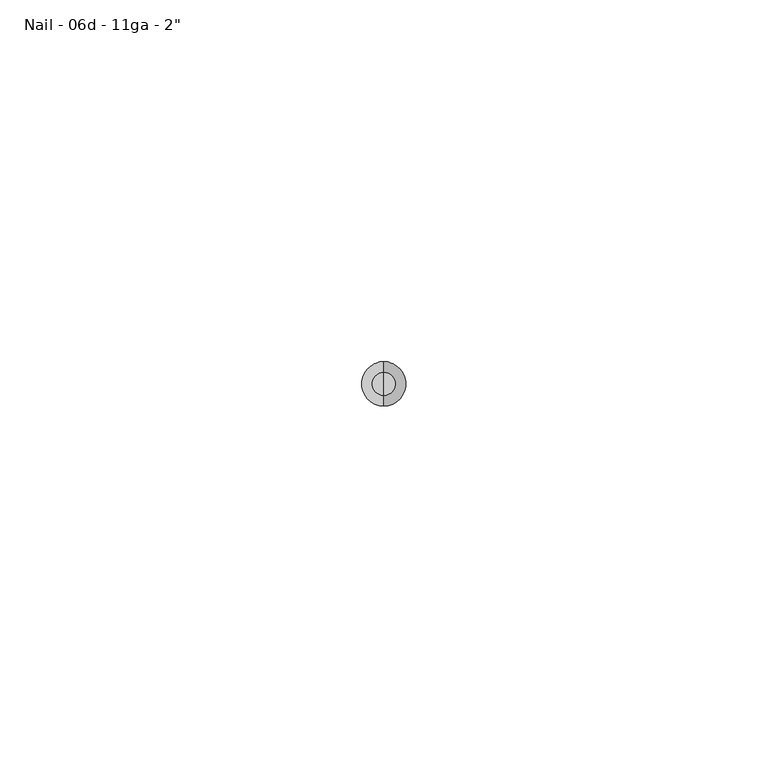
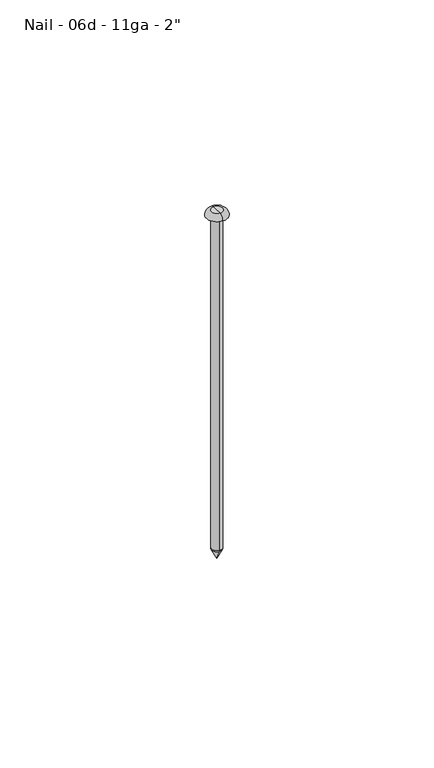
"""IFC4 building model written with IfcOpenShell, lengths in millimetres: fastener geometry."""

from ifc_helpers import new_model, si_unit, point, frame, origin, origin_2d, place, context, project, spatial, polyline, circle_curve, ellipse_curve, trimmed, segment, composite_curve, outline, extrude, source, transform, mapped, element, save
from ifc_brep_helpers import plane_surface, revolved_surface, advanced_brep


def fastener_73949ac7(model_context):
    return source(origin(), model_context, "Body", "SolidModel", [
        advanced_brep(
        [(0.0, -1.524, -101.6), (0.0, 1.524, -101.6), (0.0, 0.0, -101.6), (0.0, 0.0, -104.648)],
        [
            (0, 1, circle_curve(frame((0.0, 0.0, -101.6), z_axis=(0.0, 0.0, 1.0), x_axis=(0.0, 1.0, 0.0)), 1.524)),
            (1, 2),
            (2, 0),
            (1, 0, circle_curve(frame((0.0, 0.0, -101.6), z_axis=(0.0, 0.0, 1.0), x_axis=(0.0, 1.0, 0.0)), 1.524)),
            (3, 1),
            (0, 3),
        ],
        [
            plane_surface(frame((0.0, 0.0, -101.6), z_axis=(0.0, 0.0, 1.0), x_axis=(0.0, 1.0, 0.0))),
            revolved_surface(polyline([(0.0, 1.524, -101.6), (0.0, 0.0, -104.648)]), (0.0, 0.0, -103.0840259), (0.0, 0.0, -1.0)),
        ],
        [
            (0, [[1, 2, 3]]),
            (0, [[4, -3, -2]]),
            (1, [[5, -1, 6]]),
            (1, [[-6, -4, -5]]),
        ],
    ),
        advanced_brep(
        [(0.0, 3.048, 0.0), (0.0, -3.048, 0.0), (0.0, 0.0, 0.0), (0.0, 0.0, 1.524), (0.0, -1.5875, 1.524), (0.0, 1.5875, 1.524)],
        [
            (0, 1, circle_curve(frame((0.0, 0.0, 0.0), z_axis=(0.0, 0.0, -1.0), x_axis=(0.0, -1.0, 0.0)), 3.048)),
            (1, 2),
            (2, 0),
            (1, 0, circle_curve(frame((0.0, 0.0, 0.0), z_axis=(0.0, 0.0, -1.0), x_axis=(0.0, -1.0, 0.0)), 3.048)),
            (3, 4),
            (4, 5, circle_curve(frame((0.0, 0.0, 1.524), z_axis=(0.0, 0.0, 1.0), x_axis=(0.0, -1.0, 0.0)), 1.5875)),
            (5, 3),
            (5, 4, circle_curve(frame((0.0, 0.0, 1.524), z_axis=(0.0, 0.0, 1.0), x_axis=(0.0, -1.0, 0.0)), 1.5875)),
            (4, 1, circle_curve(frame((0.0, -1.5875, 0.0621771), z_axis=(1.0, 0.0, 0.0), x_axis=(0.0, -1.0, 0.0)), 1.4618229)),
            (0, 5, circle_curve(frame((0.0, 1.5875, 0.0621771), z_axis=(1.0, 0.0, 0.0), x_axis=(0.0, 1.0, 0.0)), 1.4618229)),
        ],
        [
            plane_surface(frame((0.0, 0.0, 0.0), z_axis=(0.0, 0.0, -1.0), x_axis=(0.0, -1.0, 0.0))),
            plane_surface(frame((0.0, 0.0, 1.524), z_axis=(0.0, 0.0, 1.0), x_axis=(0.0, -1.0, 0.0))),
            revolved_surface(trimmed(ellipse_curve(frame((0.0, -1.5875, 0.0621771), z_axis=(-1.0, 0.0, 0.0), x_axis=(0.0, -1.0, 0.0)), 1.4618229, 1.4618229), [point((0.0, -3.048, 0.0))], [point((0.0, -1.5875, 1.524))], True, "CARTESIAN"), (0.0, 0.0, 1.4840259), (0.0, 0.0, 1.0)),
        ],
        [
            (0, [[1, 2, 3]]),
            (0, [[4, -3, -2]]),
            (1, [[5, 6, 7]]),
            (1, [[-7, 8, -5]]),
            (2, [[-6, 9, -1, 10]]),
            (2, [[-8, -10, -4, -9]]),
        ],
    ),
        extrude(outline(composite_curve([segment(trimmed(circle_curve(origin_2d(), 1.524), [point((0.0, -1.524))], [point((0.0, 1.524))], False, "CARTESIAN"), True, "CONTINUOUS"), segment(trimmed(circle_curve(origin_2d(), 1.524), [point((0.0, 1.524))], [point((0.0, -1.524))], False, "CARTESIAN"), True, "CONTINUOUS")], self_intersect=False)), frame((0.0, 0.0, -101.6), z_axis=(0.0, 0.0, 1.0), x_axis=(1.0, 0.0, 0.0)), (0.0, 0.0, 1.0), 101.6),
    ])


if __name__ == "__main__":
    model = new_model("IFC4")
    model_context = context("Model", 3, world=origin())
    ifc_project = project(units=[si_unit("LENGTHUNIT", "METRE", prefix="MILLI")], contexts=[model_context])
    site = spatial("IfcSite", under=ifc_project)
    building = spatial("IfcBuilding", under=site)
    placement = place(None, origin())
    fastener_shape = fastener_73949ac7(model_context)
    element("IfcFastener", 1, ObjectType="060523 - W_P_C - Fastenings - Generic : Nail - 06d - 11ga - 2\"", at=placement, inside=building, context=model_context, shape_type="MappedRepresentation", body=[
        mapped(fastener_shape, transform((0.0, 0.0, 0.0), x_axis=(1.0, 0.0, 0.0), y_axis=(0.0, 1.0, 0.0), z_axis=(0.0, 0.0, 1.0))),
    ])
    save(model, "model.ifc")

# Revit data of these elements
# Type "060523 - W_P_C - Fastenings - Generic : Nail - 06d - 11ga - 2\""
#   Washer_Thickness = 0' - 0.00333"
#   Washer Radius = 0' - 0.07"
#   Washer Offset - Head = 0' - 0"
#   Washer Offset = 0' - 0"
#   Thickness_of_Substrate [instance default] = 0' - 1"
#   Side = 0' - 0 37/64"
#   Radius = 0' - 0.06"
#   Length [instance default] = 0' - 2"
#   Head Size = 0' - 1"
#   Head Radius = 0' - 0 1/2"
#   Head Height = 0' - 0.01"
#   Double Diameter = 0' - 0.24"
#   Diameter = 0' - 0.12"
#   Default Elevation = 4' - 0"
#   Washer_Nut_Visibility = no
#   Washer_Head_Visibility = no
#   Round_Head_Visibility = yes
#   Point Visibility = yes
#   Nut_Visibility = no
#   Hex_Head_Visiblilty = no
#   Washer Material = none
#   Bolt Material (Size) = AT SILL - FASTENER AT 24" O.C.
# Element 1 (IfcFastener, "060523 - W_P_C - Fastenings - Generic : Nail - 06d - 11ga - 2\"")
#   Length = 0' - 4"
#   Materials on its faces: "AT SILL - FASTENER AT 24\" O.C."
# Materials
#   "AT SILL - FASTENER AT 24\" O.C.": class "Generic", colour RGB 120 120 120, transparency 0, Cost = 0
